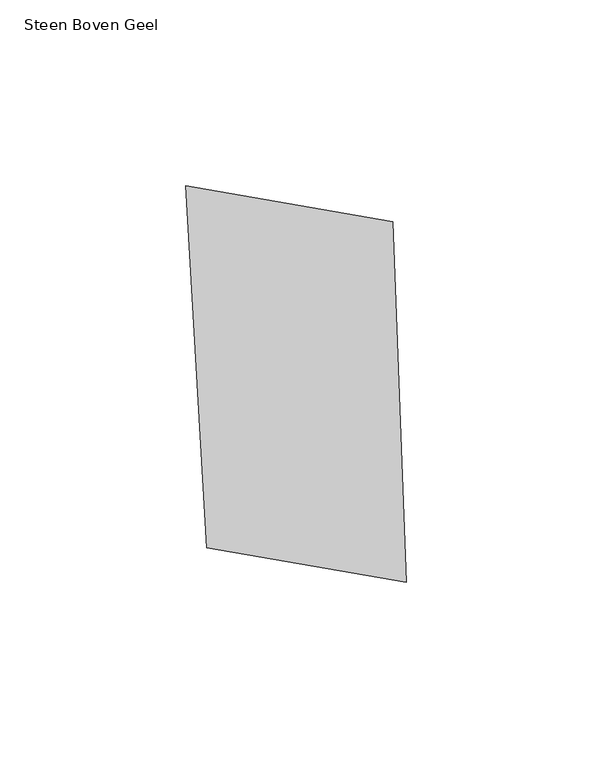
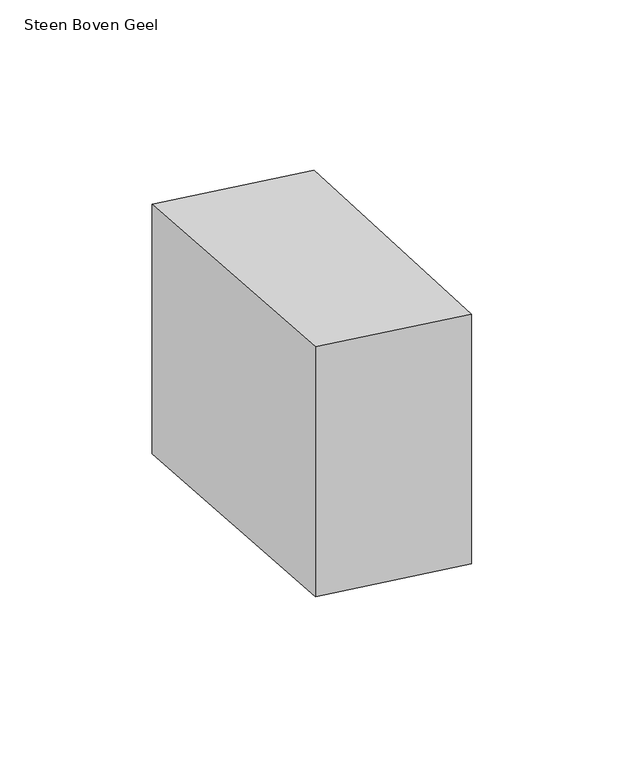
"""IFC4 building model written with IfcOpenShell, lengths in millimetres: proxy geometry, 00_GMA_steen_versie_4 : Steen Boven Geel."""

import ifcopenshell
import ifcopenshell.guid

model = None  # the IFC model being written
_history = None  # IfcOwnerHistory: only IFC2X3 demands one
_inside = {}  # id of a spatial element -> (the spatial element, [elements in it])
_under = {}  # id of a project, library or spatial element -> (it, [spatial elements below it])
_declared = {}  # id of a project -> (the project, [libraries it declares])
_typed = {}  # id of a type object -> (the type object, [elements of that type])
_made_of = {}  # id of a material, layer set ... -> (it, [elements and type objects made of it])


def new_model(schema):
    """Start an empty IFC model of exactly this schema.

    Asked for "IFC4X3", IfcOpenShell would pick the latest addendum, in which some entities
    have other attributes; the version numbers below select the first issue.
    IFC2X3 requires an IfcOwnerHistory on every rooted entity: one is made here for all.
    """
    global model, _history
    if schema == "IFC4X3":
        model = ifcopenshell.file(schema_version=(4, 3, 0, 0))
    else:
        model = ifcopenshell.file(schema=schema)
    _inside.clear()
    _under.clear()
    _declared.clear()
    _typed.clear()
    _made_of.clear()
    _history = None
    if model.schema == "IFC2X3":
        org = make("IfcOrganization", Name="unknown")
        user = make(
            "IfcPersonAndOrganization",
            ThePerson=make("IfcPerson", FamilyName="unknown"),
            TheOrganization=org,
        )
        app = make(
            "IfcApplication",
            ApplicationDeveloper=org,
            Version="unknown",
            ApplicationFullName="unknown",
            ApplicationIdentifier="unknown",
        )
        _history = make(
            "IfcOwnerHistory",
            OwningUser=user,
            OwningApplication=app,
            ChangeAction="ADDED",
            CreationDate=0,
        )
    return model


def make(cls, **values):
    """One entity of the class cls with the attributes given. An attribute that is None is left unset."""
    return model.create_entity(
        cls, **{name: value for name, value in values.items() if value is not None}
    )


def rooted(cls, **values):
    """An entity with a GlobalId (a new one), such as an element, a storey or a relation."""
    return make(cls, GlobalId=ifcopenshell.guid.new(), OwnerHistory=_history, **values)


def si_unit(unit_type, name, prefix=None):
    """IfcSIUnit, for example si_unit("LENGTHUNIT", "METRE", prefix="MILLI")."""
    return make("IfcSIUnit", UnitType=unit_type, Prefix=prefix, Name=name)


def assignment(units):
    """IfcUnitAssignment: the units of a project."""
    return None if units is None else make("IfcUnitAssignment", Units=units)


def point(xyz):
    """IfcCartesianPoint."""
    return None if xyz is None else make("IfcCartesianPoint", Coordinates=xyz)


def direction(xyz):
    """IfcDirection."""
    return None if xyz is None else make("IfcDirection", DirectionRatios=xyz)


def frame(location, z_axis=None, x_axis=None):
    """IfcAxis2Placement3D, a coordinate frame: its origin and axes. An axis left out is left unset."""
    return make(
        "IfcAxis2Placement3D",
        Location=point(location),
        Axis=direction(z_axis),
        RefDirection=direction(x_axis),
    )


def origin():
    """The frame at (0, 0, 0) with its axes left unset."""
    return frame((0.0, 0.0, 0.0))


def origin_with_axes():
    """The frame at (0, 0, 0) with the z axis (0, 0, 1) and the x axis (1, 0, 0) written out."""
    return frame((0.0, 0.0, 0.0), z_axis=(0.0, 0.0, 1.0), x_axis=(1.0, 0.0, 0.0))


def place(relative_to, where):
    """IfcLocalPlacement: puts the frame where relative to a parent placement (None: the world)."""
    return make(
        "IfcLocalPlacement", PlacementRelTo=relative_to, RelativePlacement=where
    )


def context(
    kind, dimensions, precision=None, world=None, true_north=None, identifier=None
):
    """IfcGeometricRepresentationContext, for example the 3D "Model" context."""
    return make(
        "IfcGeometricRepresentationContext",
        ContextIdentifier=identifier,
        ContextType=kind,
        CoordinateSpaceDimension=dimensions,
        Precision=precision,
        WorldCoordinateSystem=world,
        TrueNorth=true_north,
    )


def project(units=None, contexts=None):
    """IfcProject with its units and contexts."""
    return rooted(
        "IfcProject",
        Name="project",
        RepresentationContexts=contexts,
        UnitsInContext=assignment(units),
    )


def spatial(cls, under=None, at=None, **own):
    """A site, building, storey or space (cls), placed at a placement, below another one or the project."""
    s = rooted(cls, ObjectPlacement=at, **own)
    if under is not None:
        _under.setdefault(under.id(), (under, []))[1].append(s)
    return s


def polyline(points):
    """IfcPolyline through the points."""
    return make("IfcPolyline", Points=[point(p) for p in points])


def outline(outer, holes=None, kind="AREA"):
    """IfcArbitraryClosedProfileDef: a profile drawn as a closed curve; with holes, ...WithVoids."""
    if holes is None:
        return make("IfcArbitraryClosedProfileDef", ProfileType=kind, OuterCurve=outer)
    return make(
        "IfcArbitraryProfileDefWithVoids",
        ProfileType=kind,
        OuterCurve=outer,
        InnerCurves=holes,
    )


def extrude(swept, where, along, depth):
    """IfcExtrudedAreaSolid: the profile swept, set in the frame where, extruded along a direction by depth."""
    return make(
        "IfcExtrudedAreaSolid",
        SweptArea=swept,
        Position=where,
        ExtrudedDirection=direction(along),
        Depth=depth,
    )


def shape(context_of_items, identifier, shape_type, items):
    """IfcShapeRepresentation: the items that make up one representation, for example the "Body"."""
    return make(
        "IfcShapeRepresentation",
        ContextOfItems=context_of_items,
        RepresentationIdentifier=identifier,
        RepresentationType=shape_type,
        Items=items,
    )


def source(mapping_origin, context_of_items, identifier, shape_type, items):
    """IfcRepresentationMap: a shape defined once, which mapped items show again and again."""
    return make(
        "IfcRepresentationMap",
        MappingOrigin=mapping_origin,
        MappedRepresentation=shape(context_of_items, identifier, shape_type, items),
    )


def transform(
    local_origin,
    x_axis=None,
    y_axis=None,
    z_axis=None,
    scale=None,
    scale2=None,
    scale3=None,
    uniform=True,
):
    """IfcCartesianTransformationOperator3D, or its non-uniform kind. x_axis, y_axis, z_axis: its Axis1, 2, 3."""
    if uniform:
        return make(
            "IfcCartesianTransformationOperator3D",
            Axis1=direction(x_axis),
            Axis2=direction(y_axis),
            LocalOrigin=point(local_origin),
            Scale=scale,
            Axis3=direction(z_axis),
        )
    return make(
        "IfcCartesianTransformationOperator3DnonUniform",
        Axis1=direction(x_axis),
        Axis2=direction(y_axis),
        LocalOrigin=point(local_origin),
        Scale=scale,
        Axis3=direction(z_axis),
        Scale2=scale2,
        Scale3=scale3,
    )


def mapped(mapping_source, mapping_target):
    """IfcMappedItem: shows the shape of a source again, moved by a transform."""
    return make(
        "IfcMappedItem", MappingSource=mapping_source, MappingTarget=mapping_target
    )


def made_of(thing, what):
    """Note that an element or type object is made of a material, layer set ...; save() writes the relation."""
    if what is not None:
        _made_of.setdefault(what.id(), (what, []))[1].append(thing)
    return thing


def element(
    cls,
    number,
    at=None,
    inside=None,
    cuts=None,
    type_object=None,
    material=None,
    context=None,
    identifier="Body",
    shape_type=None,
    held_by="IfcProductDefinitionShape",
    body=None,
    shapes=None,
    **own,
):
    """One element of the class cls, such as IfcWall. Its Tag is "e" and its number.

    at: its placement. inside: the storey or other place that contains it. cuts: it is an
    opening in that element (IfcRelVoidsElement). A single representation is given by context,
    identifier, shape_type and body (its items); several are given by shapes. held_by: the class
    of the entity that holds the representations. save() writes the other relations.
    """
    e = rooted(cls, Tag="e%d" % number, ObjectPlacement=at, **own)
    if body is not None:
        shapes = [shape(context, identifier, shape_type, body)]
    if shapes is not None:
        e.Representation = make(held_by, Representations=shapes)
    if inside is not None:
        _inside.setdefault(inside.id(), (inside, []))[1].append(e)
    if cuts is not None:
        rooted(
            "IfcRelVoidsElement", RelatingBuildingElement=cuts, RelatedOpeningElement=e
        )
    if type_object is not None:
        _typed.setdefault(type_object.id(), (type_object, []))[1].append(e)
    return made_of(e, material)


def aggregate(whole, parts):
    """IfcRelAggregates: a whole, such as a stair, and the parts it consists of."""
    return rooted("IfcRelAggregates", RelatingObject=whole, RelatedObjects=parts)


def save(model, path):
    """Write the relations noted so far, then the file.

    IfcRelAggregates (storeys below a building ...), IfcRelContainedInSpatialStructure (elements
    in a storey), IfcRelDefinesByType, IfcRelAssociatesMaterial and IfcRelDeclares: one each for
    every whole, place, type object, material and project.
    """
    for whole, parts in _under.values():
        aggregate(whole, parts)
    for where, things in _inside.values():
        rooted(
            "IfcRelContainedInSpatialStructure",
            RelatedElements=things,
            RelatingStructure=where,
        )
    for kind, things in _typed.values():
        rooted("IfcRelDefinesByType", RelatedObjects=things, RelatingType=kind)
    for what, things in _made_of.values():
        rooted("IfcRelAssociatesMaterial", RelatedObjects=things, RelatingMaterial=what)
    for by, libraries in _declared.values():
        rooted("IfcRelDeclares", RelatingContext=by, RelatedDefinitions=libraries)
    model.write(path)


def steen_boven_geel_bff6007e(model_context):
    return source(origin(), model_context, "Body", "SweptSolid", [
        extrude(outline(polyline([(98.7689498, 120.5188388), (102.3022786, 23.3772311), (48.5532041, 32.6777689), (42.9354805, 130.2005135), (98.7689498, 120.5188388)])), origin_with_axes(), (0.0, 0.0, 1.0), 100.0),
    ])


if __name__ == "__main__":
    model = new_model("IFC4")
    model_context = context("Model", 3, world=origin())
    ifc_project = project(units=[si_unit("LENGTHUNIT", "METRE", prefix="MILLI")], contexts=[model_context])
    site = spatial("IfcSite", under=ifc_project)
    building = spatial("IfcBuilding", under=site)
    placement = place(None, origin())
    steen_boven_geel_shape = steen_boven_geel_bff6007e(model_context)
    element("IfcBuildingElementProxy", 1, Name="00_GMA_steen_versie_4 : Steen Boven Geel", ObjectType="00_GMA_steen_versie_4 : Steen Boven Geel", at=placement, inside=building, context=model_context, shape_type="MappedRepresentation", body=[
        mapped(steen_boven_geel_shape, transform((0.0, 0.0, 0.0), x_axis=(1.0, 0.0, 0.0), y_axis=(0.0, 1.0, 0.0), z_axis=(0.0, 0.0, 1.0))),
    ])
    save(model, "model.ifc")

# Revit data of these elements
# Type "00_GMA_steen_versie_4 : Steen Boven Geel"
#   StootVoegHalfBoven [instance default] = 5 mm
#   StootVoegHalf [instance default] = 5 mm
#   StootVoegBreedteOnder = 10 mm
#   StootVoegBreedteBoven = 10 mm
#   Steendikte = 100 mm
#   LintVoegOnderHalf = 5 mm
#   LintVoegOnder = 10 mm
#   LintVoegBovenHalf = 0 mm
#   LintVoegBoven = 0 mm
#   materiaal = 21_steen_geel
#   MateriaalVoeg = none
#   Default Elevation = 0
# Element 1 (IfcBuildingElementProxy, "00_GMA_steen_versie_4 : Steen Boven Geel")
#   Materials on its faces: "21_steen_geel"
# Materials
#   "21_steen_geel": class "Unassigned", colour RGB 202 202 0, transparency 0, Cost = 0
